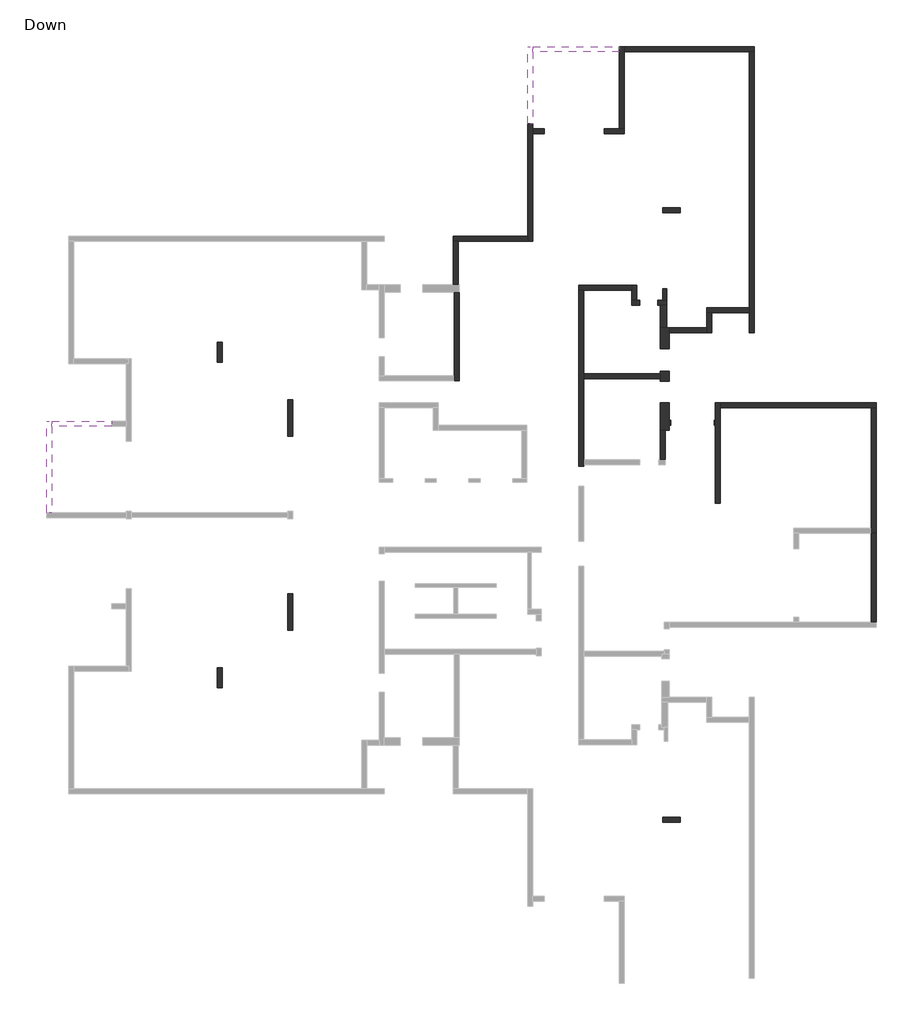
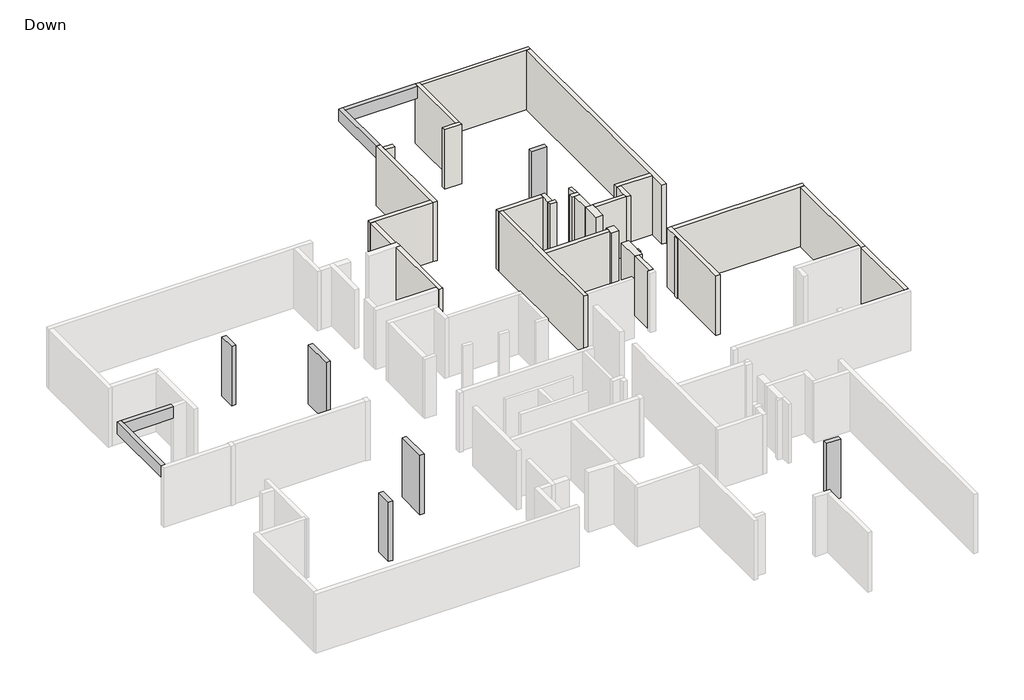
# One storey, part 3 of 3: 30 walls, 6 columns, 4 beams.
# Revit data of these elements (continued)
# Element 35 (IfcWall, "20") (continued)
#   Phase Created = New Construction
#   Base Constraint = Down
#   Top Constraint = Typical Floor
#   Materials on its faces: "Concrete"
# Element 36 (IfcWall, "20")
#   Comments = ""
#   Mark = "W77"
#   SOFiSTiK_EdgeZones = "W77"
#   SOFiSTiK_AMG_Comments = ""
#   Top Offset = 0 cm
#   Base Offset = 0 cm
#   wall height = 300 cm
#   SOFiSTiK_AMG_Scheduled = yes
#   SOFiSTiK_AMG_Adjusted = yes
#   Phase Created = New Construction
#   Base Constraint = Down
#   Top Constraint = Typical Floor
#   Materials on its faces: "Concrete"
# Element 37 (IfcWall, "25")
#   Comments = ""
#   Mark = "W97"
#   SOFiSTiK_EdgeZones = "W97"
#   SOFiSTiK_AMG_Comments = ""
#   Top Offset = 0 cm
#   Base Offset = 0 cm
#   wall height = 300 cm
#   SOFiSTiK_AMG_Scheduled = yes
#   SOFiSTiK_AMG_Adjusted = yes
#   Phase Created = New Construction
#   Base Constraint = Down
#   Top Constraint = Typical Floor
#   Materials on its faces: "Concrete"
# Element 38 (IfcWall, "35")
#   Comments = ""
#   Mark = "W94"
#   SOFiSTiK_EdgeZones = "W94"
#   SOFiSTiK_AMG_Comments = ""
#   Top Offset = 0 cm
#   Base Offset = 0 cm
#   wall height = 300 cm
#   SOFiSTiK_AMG_Scheduled = yes
#   SOFiSTiK_AMG_Adjusted = yes
#   Phase Created = New Construction
#   Base Constraint = Down
#   Top Constraint = Typical Floor
#   Materials on its faces: "Concrete"
# Element 39 (IfcWall, "35")
#   Comments = ""
#   Mark = "W95"
#   SOFiSTiK_EdgeZones = "W95"
#   SOFiSTiK_AMG_Comments = ""
#   Top Offset = 0 cm
#   Base Offset = 0 cm
#   wall height = 300 cm
#   SOFiSTiK_AMG_Scheduled = yes
#   SOFiSTiK_AMG_Adjusted = yes
#   Phase Created = New Construction
#   Base Constraint = Down
#   Top Constraint = Typical Floor
#   Materials on its faces: "Concrete"
# Element 40 (IfcWall, "35")
#   Comments = ""
#   Mark = "W96"
#   SOFiSTiK_EdgeZones = "W96"
#   SOFiSTiK_AMG_Comments = ""
#   Top Offset = 0 cm
#   Base Offset = 0 cm
#   wall height = 300 cm
#   SOFiSTiK_AMG_Scheduled = yes
#   SOFiSTiK_AMG_Adjusted = yes
#   Phase Created = New Construction
#   Base Constraint = Down
#   Top Constraint = Typical Floor
#   Materials on its faces: "Concrete"
# Materials
#   "Concrete": class "Concrete", colour RGB 192 192 192, transparency 0, Keynote = "01000", Description = "Cast-in-place concrete", Cost = 0
